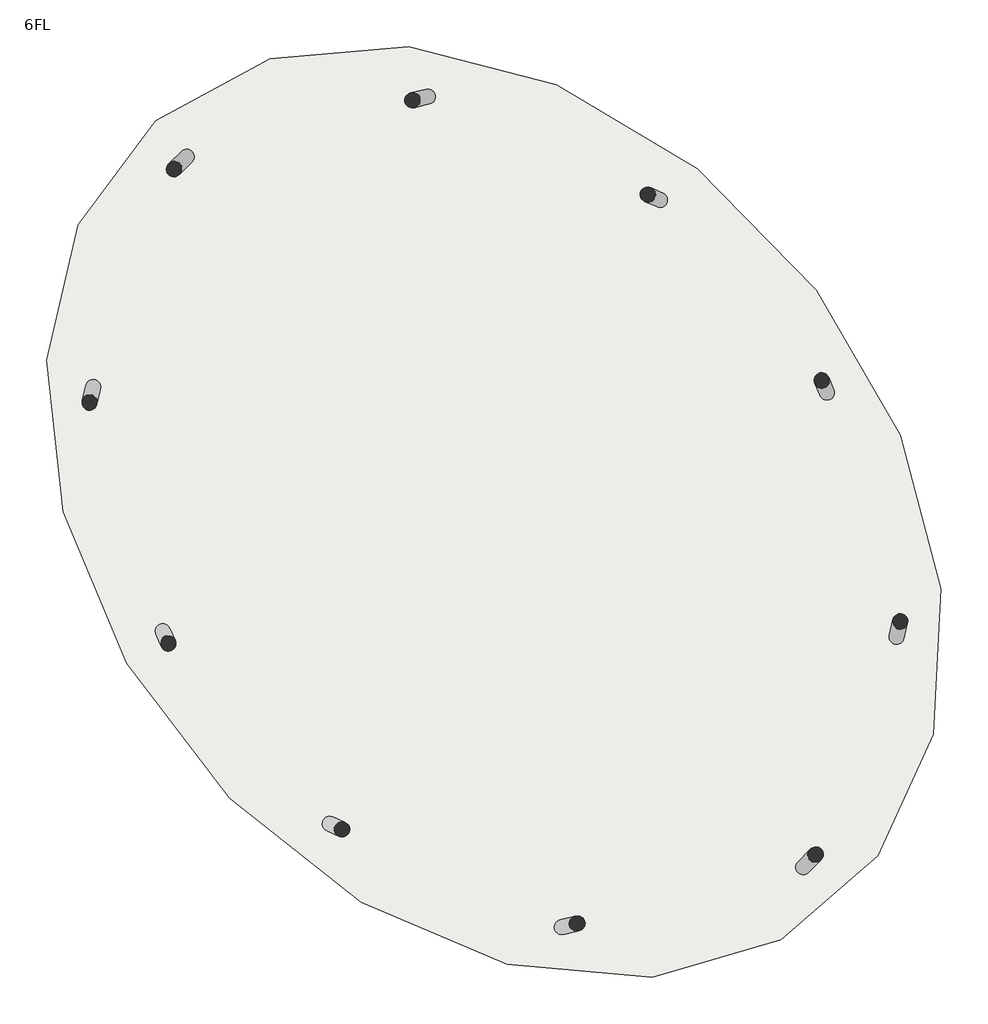
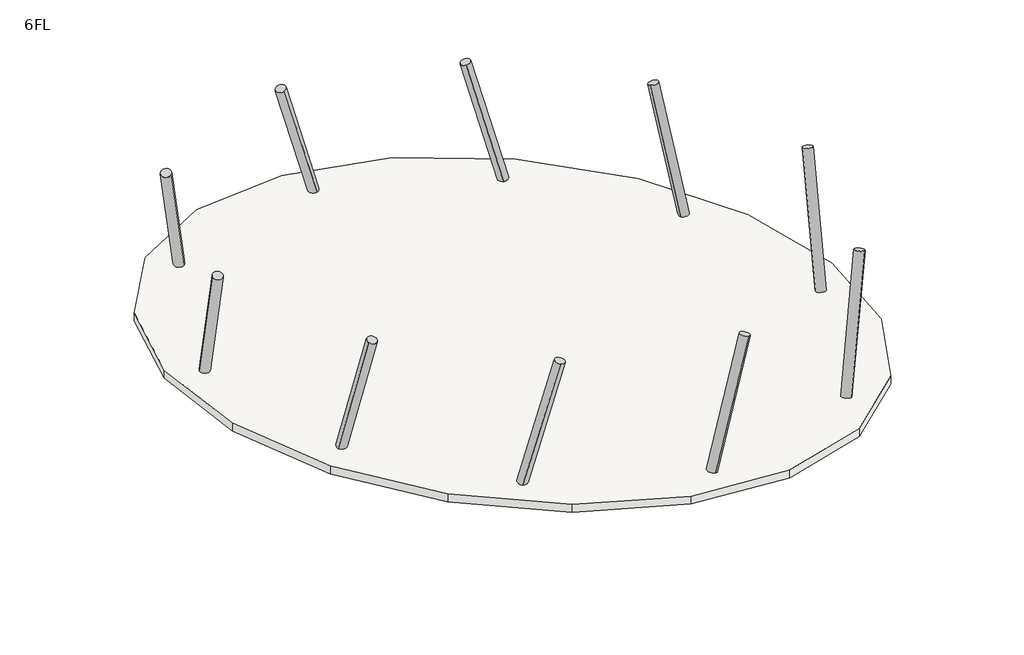
# One storey: 10 columns, 1 slab.
"""IFC4 building model written with IfcOpenShell, lengths in millimetres."""

import ifcopenshell
import ifcopenshell.guid

model = None  # the IFC model being written
_history = None  # IfcOwnerHistory: only IFC2X3 demands one
_inside = {}  # id of a spatial element -> (the spatial element, [elements in it])
_under = {}  # id of a project, library or spatial element -> (it, [spatial elements below it])
_declared = {}  # id of a project -> (the project, [libraries it declares])
_typed = {}  # id of a type object -> (the type object, [elements of that type])
_made_of = {}  # id of a material, layer set ... -> (it, [elements and type objects made of it])


def new_model(schema):
    """Start an empty IFC model of exactly this schema.

    Asked for "IFC4X3", IfcOpenShell would pick the latest addendum, in which some entities
    have other attributes; the version numbers below select the first issue.
    IFC2X3 requires an IfcOwnerHistory on every rooted entity: one is made here for all.
    """
    global model, _history
    if schema == "IFC4X3":
        model = ifcopenshell.file(schema_version=(4, 3, 0, 0))
    else:
        model = ifcopenshell.file(schema=schema)
    _inside.clear()
    _under.clear()
    _declared.clear()
    _typed.clear()
    _made_of.clear()
    _history = None
    if model.schema == "IFC2X3":
        org = make("IfcOrganization", Name="unknown")
        user = make(
            "IfcPersonAndOrganization",
            ThePerson=make("IfcPerson", FamilyName="unknown"),
            TheOrganization=org,
        )
        app = make(
            "IfcApplication",
            ApplicationDeveloper=org,
            Version="unknown",
            ApplicationFullName="unknown",
            ApplicationIdentifier="unknown",
        )
        _history = make(
            "IfcOwnerHistory",
            OwningUser=user,
            OwningApplication=app,
            ChangeAction="ADDED",
            CreationDate=0,
        )
    return model


def make(cls, **values):
    """One entity of the class cls with the attributes given. An attribute that is None is left unset."""
    return model.create_entity(
        cls, **{name: value for name, value in values.items() if value is not None}
    )


def rooted(cls, **values):
    """An entity with a GlobalId (a new one), such as an element, a storey or a relation."""
    return make(cls, GlobalId=ifcopenshell.guid.new(), OwnerHistory=_history, **values)


def si_unit(unit_type, name, prefix=None):
    """IfcSIUnit, for example si_unit("LENGTHUNIT", "METRE", prefix="MILLI")."""
    return make("IfcSIUnit", UnitType=unit_type, Prefix=prefix, Name=name)


def assignment(units):
    """IfcUnitAssignment: the units of a project."""
    return None if units is None else make("IfcUnitAssignment", Units=units)


def point(xyz):
    """IfcCartesianPoint."""
    return None if xyz is None else make("IfcCartesianPoint", Coordinates=xyz)


def direction(xyz):
    """IfcDirection."""
    return None if xyz is None else make("IfcDirection", DirectionRatios=xyz)


def frame(location, z_axis=None, x_axis=None):
    """IfcAxis2Placement3D, a coordinate frame: its origin and axes. An axis left out is left unset."""
    return make(
        "IfcAxis2Placement3D",
        Location=point(location),
        Axis=direction(z_axis),
        RefDirection=direction(x_axis),
    )


def frame_2d(location, x_axis=None):
    """IfcAxis2Placement2D, a coordinate frame in the plane: its origin and x axis."""
    return make(
        "IfcAxis2Placement2D", Location=point(location), RefDirection=direction(x_axis)
    )


def origin():
    """The frame at (0, 0, 0) with its axes left unset."""
    return frame((0.0, 0.0, 0.0))


def place(relative_to, where):
    """IfcLocalPlacement: puts the frame where relative to a parent placement (None: the world)."""
    return make(
        "IfcLocalPlacement", PlacementRelTo=relative_to, RelativePlacement=where
    )


def context(
    kind, dimensions, precision=None, world=None, true_north=None, identifier=None
):
    """IfcGeometricRepresentationContext, for example the 3D "Model" context."""
    return make(
        "IfcGeometricRepresentationContext",
        ContextIdentifier=identifier,
        ContextType=kind,
        CoordinateSpaceDimension=dimensions,
        Precision=precision,
        WorldCoordinateSystem=world,
        TrueNorth=true_north,
    )


def project(units=None, contexts=None):
    """IfcProject with its units and contexts."""
    return rooted(
        "IfcProject",
        Name="project",
        RepresentationContexts=contexts,
        UnitsInContext=assignment(units),
    )


def spatial(cls, under=None, at=None, **own):
    """A site, building, storey or space (cls), placed at a placement, below another one or the project."""
    s = rooted(cls, ObjectPlacement=at, **own)
    if under is not None:
        _under.setdefault(under.id(), (under, []))[1].append(s)
    return s


def polyline(points):
    """IfcPolyline through the points."""
    return make("IfcPolyline", Points=[point(p) for p in points])


def circle_curve(where, radius):
    """IfcCircle in the frame where."""
    return make("IfcCircle", Position=where, Radius=radius)


def trimmed(basis, trim1, trim2, sense, master):
    """IfcTrimmedCurve: the piece of a basis curve between two trims."""
    return make(
        "IfcTrimmedCurve",
        BasisCurve=basis,
        Trim1=trim1,
        Trim2=trim2,
        SenseAgreement=sense,
        MasterRepresentation=master,
    )


def segment(curve, same_sense, transition):
    """IfcCompositeCurveSegment."""
    return make(
        "IfcCompositeCurveSegment",
        Transition=transition,
        SameSense=same_sense,
        ParentCurve=curve,
    )


def composite_curve(segments, self_intersect=None):
    """IfcCompositeCurve: segments joined end to end."""
    return make("IfcCompositeCurve", Segments=segments, SelfIntersect=self_intersect)


def outline(outer, holes=None, kind="AREA"):
    """IfcArbitraryClosedProfileDef: a profile drawn as a closed curve; with holes, ...WithVoids."""
    if holes is None:
        return make("IfcArbitraryClosedProfileDef", ProfileType=kind, OuterCurve=outer)
    return make(
        "IfcArbitraryProfileDefWithVoids",
        ProfileType=kind,
        OuterCurve=outer,
        InnerCurves=holes,
    )


def extrude(swept, where, along, depth):
    """IfcExtrudedAreaSolid: the profile swept, set in the frame where, extruded along a direction by depth."""
    return make(
        "IfcExtrudedAreaSolid",
        SweptArea=swept,
        Position=where,
        ExtrudedDirection=direction(along),
        Depth=depth,
    )


def shape(context_of_items, identifier, shape_type, items):
    """IfcShapeRepresentation: the items that make up one representation, for example the "Body"."""
    return make(
        "IfcShapeRepresentation",
        ContextOfItems=context_of_items,
        RepresentationIdentifier=identifier,
        RepresentationType=shape_type,
        Items=items,
    )


def made_of(thing, what):
    """Note that an element or type object is made of a material, layer set ...; save() writes the relation."""
    if what is not None:
        _made_of.setdefault(what.id(), (what, []))[1].append(thing)
    return thing


def element(
    cls,
    number,
    at=None,
    inside=None,
    cuts=None,
    type_object=None,
    material=None,
    context=None,
    identifier="Body",
    shape_type=None,
    held_by="IfcProductDefinitionShape",
    body=None,
    shapes=None,
    **own,
):
    """One element of the class cls, such as IfcWall. Its Tag is "e" and its number.

    at: its placement. inside: the storey or other place that contains it. cuts: it is an
    opening in that element (IfcRelVoidsElement). A single representation is given by context,
    identifier, shape_type and body (its items); several are given by shapes. held_by: the class
    of the entity that holds the representations. save() writes the other relations.
    """
    e = rooted(cls, Tag="e%d" % number, ObjectPlacement=at, **own)
    if body is not None:
        shapes = [shape(context, identifier, shape_type, body)]
    if shapes is not None:
        e.Representation = make(held_by, Representations=shapes)
    if inside is not None:
        _inside.setdefault(inside.id(), (inside, []))[1].append(e)
    if cuts is not None:
        rooted(
            "IfcRelVoidsElement", RelatingBuildingElement=cuts, RelatedOpeningElement=e
        )
    if type_object is not None:
        _typed.setdefault(type_object.id(), (type_object, []))[1].append(e)
    return made_of(e, material)


def aggregate(whole, parts):
    """IfcRelAggregates: a whole, such as a stair, and the parts it consists of."""
    return rooted("IfcRelAggregates", RelatingObject=whole, RelatedObjects=parts)


def save(model, path):
    """Write the relations noted so far, then the file.

    IfcRelAggregates (storeys below a building ...), IfcRelContainedInSpatialStructure (elements
    in a storey), IfcRelDefinesByType, IfcRelAssociatesMaterial and IfcRelDeclares: one each for
    every whole, place, type object, material and project.
    """
    for whole, parts in _under.values():
        aggregate(whole, parts)
    for where, things in _inside.values():
        rooted(
            "IfcRelContainedInSpatialStructure",
            RelatedElements=things,
            RelatingStructure=where,
        )
    for kind, things in _typed.values():
        rooted("IfcRelDefinesByType", RelatedObjects=things, RelatingType=kind)
    for what, things in _made_of.values():
        rooted("IfcRelAssociatesMaterial", RelatedObjects=things, RelatingMaterial=what)
    for by, libraries in _declared.values():
        rooted("IfcRelDeclares", RelatingContext=by, RelatedDefinitions=libraries)
    model.write(path)


model = new_model("IFC4")

# Units and contexts
model_context = context("Model", 3, world=origin())
ifc_project = project(units=[si_unit("LENGTHUNIT", "METRE", prefix="MILLI")], contexts=[model_context])

# Site, building, storey
site = spatial("IfcSite", under=ifc_project)
building = spatial("IfcBuilding", under=site)
storey = spatial("IfcBuildingStorey", under=building, Name="6FL", Elevation=22500.0)

# Columns
placement = place(None, origin())
element("IfcColumn", 1, ObjectType="コンクリート-円形-柱 : 750", at=placement, inside=storey, context=model_context, shape_type="SweptSolid", body=[
    extrude(outline(composite_curve([segment(trimmed(circle_curve(frame_2d((0.0, -175.0)), 175.0), [point((-1e-07, -350.0))], [point((0.0, 0.0))], False, "CARTESIAN"), True, "CONTINUOUS"), segment(trimmed(circle_curve(frame_2d((0.0, -175.0)), 175.0), [point((0.0, 0.0))], [point((-1e-07, -350.0))], False, "CARTESIAN"), True, "CONTINUOUS")], self_intersect=False)), frame((-7039.7311612, 8143.3469885, 22500.0), z_axis=(-0.23170722232410254, -0.23170722232407712, 0.9447875561446129), x_axis=(-0.6680656877305583, -0.6680656877304849, -0.32768349631052573)), (0.0, 0.0, 1.0), 4762.9755184),
])
element("IfcColumn", 2, ObjectType="コンクリート-円形-柱 : 750", at=placement, inside=storey, context=model_context, shape_type="SweptSolid", body=[
    extrude(outline(composite_curve([segment(trimmed(circle_curve(frame_2d((0.0, -175.0)), 175.0), [point((0.0, -350.0))], [point((0.0, 0.0))], False, "CARTESIAN"), True, "CONTINUOUS"), segment(trimmed(circle_curve(frame_2d((0.0, -175.0)), 175.0), [point((0.0, 0.0))], [point((0.0, -350.0))], False, "CARTESIAN"), True, "CONTINUOUS")], self_intersect=False)), frame((-9169.5730444, 2870.3696192, 22500.0), z_axis=(-0.06773274998007163, -0.28840793400318554, 0.9551089666546699), x_axis=(-0.21836666720260925, -0.9298113447570836, -0.2962547245460378)), (0.0, 0.0, 1.0), 4711.5042965),
])
element("IfcColumn", 3, ObjectType="コンクリート-円形-柱 : 750", at=placement, inside=storey, context=model_context, shape_type="SweptSolid", body=[
    extrude(outline(composite_curve([segment(trimmed(circle_curve(frame_2d((0.0, -175.0)), 175.0), [point((0.0, -350.0))], [point((0.0, 0.0))], False, "CARTESIAN"), True, "CONTINUOUS"), segment(trimmed(circle_curve(frame_2d((0.0, -175.0)), 175.0), [point((0.0, 0.0))], [point((0.0, -350.0))], False, "CARTESIAN"), True, "CONTINUOUS")], self_intersect=False)), frame((-7565.7209851, -2701.5135041, 22500.0), z_axis=(0.10175828080216195, -0.23038778551623762, 0.9677637731249877), x_axis=(0.39100340519329535, -0.8852587518349425, -0.2518596423146979)), (0.0, 0.0, 1.0), 4649.8950725),
])
element("IfcColumn", 4, ObjectType="コンクリート-円形-柱 : 750", at=placement, inside=storey, context=model_context, shape_type="SweptSolid", body=[
    extrude(outline(composite_curve([segment(trimmed(circle_curve(frame_2d((0.0, -175.0)), 175.0), [point((0.0, -349.9999999))], [point((0.0, 0.0))], False, "CARTESIAN"), True, "CONTINUOUS"), segment(trimmed(circle_curve(frame_2d((0.0, -175.0)), 175.0), [point((0.0, 0.0))], [point((0.0, -349.9999999))], False, "CARTESIAN"), True, "CONTINUOUS")], self_intersect=False)), frame((-3772.7924801, -7092.5556991, 22500.0), z_axis=(0.23038778669285745, -0.10175827904508689, 0.9677637730296318), x_axis=(0.8852587549809827, -0.39100339783442956, -0.2518596426811)), (0.0, 0.0, 1.0), 4649.8950725),
])
element("IfcColumn", 5, ObjectType="コンクリート-円形-柱 : 750", at=placement, inside=storey, context=model_context, shape_type="SweptSolid", body=[
    extrude(outline(composite_curve([segment(trimmed(circle_curve(frame_2d((0.0, -175.0)), 175.0), [point((0.0, -350.0))], [point((0.0, 0.0))], False, "CARTESIAN"), True, "CONTINUOUS"), segment(trimmed(circle_curve(frame_2d((0.0, -175.0)), 175.0), [point((0.0, 0.0))], [point((0.0, -350.0))], False, "CARTESIAN"), True, "CONTINUOUS")], self_intersect=False)), frame((1511.5344978, -9488.6961955, 22500.0), z_axis=(0.28840793397162084, 0.06773275301815233, 0.955108966448752), x_axis=(0.9298113423712713, 0.21836667646080446, -0.29625472520990587)), (0.0, 0.0, 1.0), 4711.5042965),
])
element("IfcColumn", 6, ObjectType="コンクリート-円形-柱 : 750", at=placement, inside=storey, context=model_context, shape_type="SweptSolid", body=[
    extrude(outline(composite_curve([segment(trimmed(circle_curve(frame_2d((0.0, -175.0)), 175.0), [point((0.0, -350.0))], [point((0.0, 0.0))], False, "CARTESIAN"), True, "CONTINUOUS"), segment(trimmed(circle_curve(frame_2d((0.0, -175.0)), 175.0), [point((0.0, 0.0))], [point((0.0, -350.0))], False, "CARTESIAN"), True, "CONTINUOUS")], self_intersect=False)), frame((7039.7311977, -8143.3469806, 22500.0), z_axis=(0.23170722195590393, 0.23170722336942046, 0.9447875559785444), x_axis=(0.6680656855753456, 0.6680656896508416, -0.32768349678933945)), (0.0, 0.0, 1.0), 4762.9755184),
])
element("IfcColumn", 7, ObjectType="コンクリート-円形-柱 : 750", at=placement, inside=storey, context=model_context, shape_type="SweptSolid", body=[
    extrude(outline(composite_curve([segment(trimmed(circle_curve(frame_2d((0.0, -174.9999999)), 175.0), [point((0.0, -349.9999999))], [point((0.0, 0.0))], False, "CARTESIAN"), True, "CONTINUOUS"), segment(trimmed(circle_curve(frame_2d((0.0, -174.9999999)), 175.0), [point((0.0, 0.0))], [point((0.0, -349.9999999))], False, "CARTESIAN"), True, "CONTINUOUS")], self_intersect=False)), frame((9169.5730409, -2870.3695973, 22500.0), z_axis=(0.06773274931987647, 0.288407933877303, 0.9551089667395004), x_axis=(0.21836666529515733, 0.9298113452921882, -0.29625472427254895)), (0.0, 0.0, 1.0), 4711.5042965),
])
element("IfcColumn", 8, ObjectType="コンクリート-円形-柱 : 750", at=placement, inside=storey, context=model_context, shape_type="SweptSolid", body=[
    extrude(outline(composite_curve([segment(trimmed(circle_curve(frame_2d((0.0, -175.0)), 175.0), [point((-1e-07, -350.0))], [point((0.0, 0.0))], False, "CARTESIAN"), True, "CONTINUOUS"), segment(trimmed(circle_curve(frame_2d((0.0, -175.0)), 175.0), [point((0.0, 0.0))], [point((-1e-07, -350.0))], False, "CARTESIAN"), True, "CONTINUOUS")], self_intersect=False)), frame((7565.7209621, 2701.5135156, 22500.0), z_axis=(-0.10175828112770693, 0.2303877848134641, 0.9677637732580608), x_axis=(-0.3910034072917814, 0.8852587510535532, -0.25185964180336734)), (0.0, 0.0, 1.0), 4649.8950725),
])
element("IfcColumn", 9, ObjectType="コンクリート-円形-柱 : 750", at=placement, inside=storey, context=model_context, shape_type="SweptSolid", body=[
    extrude(outline(composite_curve([segment(trimmed(circle_curve(frame_2d((0.0, -175.0)), 175.0), [point((0.0, -350.0))], [point((0.0, 0.0))], False, "CARTESIAN"), True, "CONTINUOUS"), segment(trimmed(circle_curve(frame_2d((0.0, -175.0)), 175.0), [point((0.0, 0.0))], [point((0.0, -350.0))], False, "CARTESIAN"), True, "CONTINUOUS")], self_intersect=False)), frame((3772.7925224, 7092.5556707, 22500.0), z_axis=(-0.23038778591581402, 0.10175828044008087, 0.9677637730679357), x_axis=(-0.8852587525475804, 0.39100340343862605, -0.2518596425339183)), (0.0, 0.0, 1.0), 4649.8950725),
])
element("IfcColumn", 10, ObjectType="コンクリート-円形-柱 : 750", at=placement, inside=storey, context=model_context, shape_type="SweptSolid", body=[
    extrude(outline(composite_curve([segment(trimmed(circle_curve(frame_2d((0.0, -175.0)), 175.0), [point((0.0, -349.9999999))], [point((0.0, 0.0))], False, "CARTESIAN"), True, "CONTINUOUS"), segment(trimmed(circle_curve(frame_2d((0.0, -175.0)), 175.0), [point((0.0, 0.0))], [point((0.0, -349.9999999))], False, "CARTESIAN"), True, "CONTINUOUS")], self_intersect=False)), frame((-1511.5344177, 9488.6961899, 22500.0), z_axis=(-0.2884079340340313, -0.06773275055527382, 0.9551089666045645), x_axis=(-0.9298113443007568, -0.21836666892650627, -0.2962547247075751)), (0.0, 0.0, 1.0), 4711.5042965),
])

# Slab
element("IfcSlab", 11, ObjectType="一般 300 mm", at=placement, inside=storey, context=model_context, shape_type="SweptSolid", body=[
    extrude(outline(polyline([(-10427.5093857, 3524.8849596), (-9684.5978157, 6673.0080781), (-7885.4229754, 9100.263229), (-5226.8245056, 10535.6906394), (-2005.0174013, 10823.0158083), (1427.9390262, 9937.1874763), (4703.1305124, 7978.5230207), (7469.8107829, 5159.7125372), (9430.9837871, 1784.0150935), (10374.6434278, -1786.5177724), (10195.6775591, -5168.7269298), (8907.4974352, -7995.9382289), (6646.8820373, -9954.7725916), (3665.1205444, -10827.486812), (291.867896, -10523.2925068), (-3108.0253329, -9081.0981746), (-6170.2590145, -6659.4752206), (-8566.6384236, -3519.7972141), (-10039.2581475, 0.8045629), (-10427.5093857, 3524.8849596)])), frame((0.0, 0.0, 22200.0), z_axis=(0.0, 0.0, 1.0), x_axis=(1.0, 0.0, 0.0)), (0.0, 0.0, 1.0), 300.0),
])

save(model, "model.ifc")

# Revit data of these elements
# Type "コンクリート-円形-柱 : 750"
#   Keynote = "03310.Q1"
#   R = 350 mm
#   Structural Material [instance default] = コンクリート - 現場打ち
# Type "一般 300 mm"
#   Function = 0
#   Layers, outside or top first: 300 mm no material (function 1)
# Elements 1, 2, 3, 4, 5, 6, 7, 8, 9, 10 (IfcColumn, "コンクリート-円形-柱 : 750")
#   Structural Material = コンクリート - 現場打ち
#   Phase Created = 新しい建設
#   Materials on its faces: "コンクリート - 現場打ち"
# Element 11 (IfcSlab, "一般 300 mm")
#   Height Offset From Level = 0 mm
#   Phase Created = 新しい建設
# Materials
#   "コンクリート - 現場打ち": class "コンクリート", colour RGB 192 192 192, transparency 0
